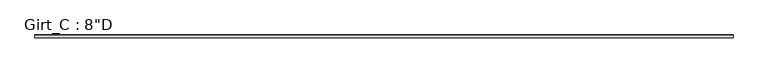
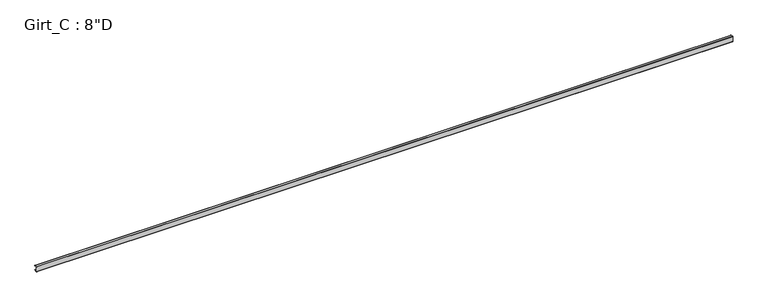
"""IFC4 building model written with IfcOpenShell, lengths in millimetres: beam geometry."""

from ifc_helpers import new_model, si_unit, point, frame, frame_2d, origin, place, context, project, spatial, polyline, circle_curve, trimmed, segment, composite_curve, outline, extrude, source, transform, mapped, element, save


def beam_eedc5fdb(model_context):
    return source(origin(), model_context, "Body", "SweptSolid", [
        extrude(outline(composite_curve([segment(polyline([(87.5109375, 101.6), (99.7560415, 87.0068534), (97.6278742, 85.221109), (86.2154765, 98.821875), (3.3005807, 98.821875)]), True, "CONTINUOUS"), segment(trimmed(circle_curve(frame_2d((3.3741066, 96.8381931)), 1.9850441), [point((3.3005807, 98.821875))], [point((1.3890625, 96.8381931))], True, "CARTESIAN"), True, "CONTINUOUS"), segment(polyline([(1.3890625, 96.8381931), (1.3890625, -96.8389339)]), True, "CONTINUOUS"), segment(trimmed(circle_curve(frame_2d((3.3748024, -96.8389339)), 1.9857399), [point((1.3890625, -96.8389339))], [point((3.2694106, -98.821875))], True, "CARTESIAN"), True, "CONTINUOUS"), segment(polyline([(3.2694106, -98.821875), (86.2154765, -98.821875), (97.6510975, -85.1934327), (99.7792647, -86.979177), (87.5109375, -101.6), (3.3734375, -101.6)]), True, "CONTINUOUS"), segment(trimmed(circle_curve(frame_2d((3.3734375, -96.8375)), 4.7625), [point((3.3734375, -101.6))], [point((-1.3890625, -96.8375))], False, "CARTESIAN"), True, "CONTINUOUS"), segment(polyline([(-1.3890625, -96.8375), (-1.3890625, 96.8375)]), True, "CONTINUOUS"), segment(trimmed(circle_curve(frame_2d((3.3734375, 96.8375)), 4.7625), [point((-1.3890625, 96.8375))], [point((3.3734375, 101.6))], False, "CARTESIAN"), True, "CONTINUOUS"), segment(polyline([(3.3734375, 101.6), (87.5109375, 101.6)]), True, "CONTINUOUS")], self_intersect=False)), frame((-12801.5873, 0.0, 0.0), z_axis=(1.0, 0.0, 0.0), x_axis=(0.0, 1.0, 0.0)), (0.0, 0.0, 1.0), 25661.239),
    ])


if __name__ == "__main__":
    model = new_model("IFC4")
    model_context = context("Model", 3, world=origin())
    ifc_project = project(units=[si_unit("LENGTHUNIT", "METRE", prefix="MILLI")], contexts=[model_context])
    site = spatial("IfcSite", under=ifc_project)
    building = spatial("IfcBuilding", under=site)
    placement = place(None, origin())
    beam_shape = beam_eedc5fdb(model_context)
    element("IfcBeam", 1, ObjectType="Girt_C : 8\"D", at=placement, inside=building, context=model_context, shape_type="MappedRepresentation", body=[
        mapped(beam_shape, transform((0.0, 0.0, 0.0), x_axis=(1.0, 0.0, 0.0), y_axis=(0.0, 1.0, 0.0), z_axis=(0.0, 0.0, 1.0))),
    ])
    save(model, "model.ifc")

# Revit data of these elements
# Type "Girt_C : 8\"D"
#   half leg = 0' - 1 3/4"
#   Web_Thickness = 0' - 0 7/64"
#   Length [instance default] = 10' - 0"
#   Leg_1 = 0' - 3 1/2"
#   Height = 0' - 8"
#   Structural Material [instance default] = none
# Element 1 (IfcBeam, "Girt_C : 8\"D")
#   Materials on its faces: "CEE' SECTION (8.0x3.5C - SEE STRUCT. DWGS)"
# Materials
#   "CEE' SECTION (8.0x3.5C - SEE STRUCT. DWGS)": class "Metal", colour RGB 137 146 153, transparency 0, Description = "Steel, mill finish", Cost = 0
